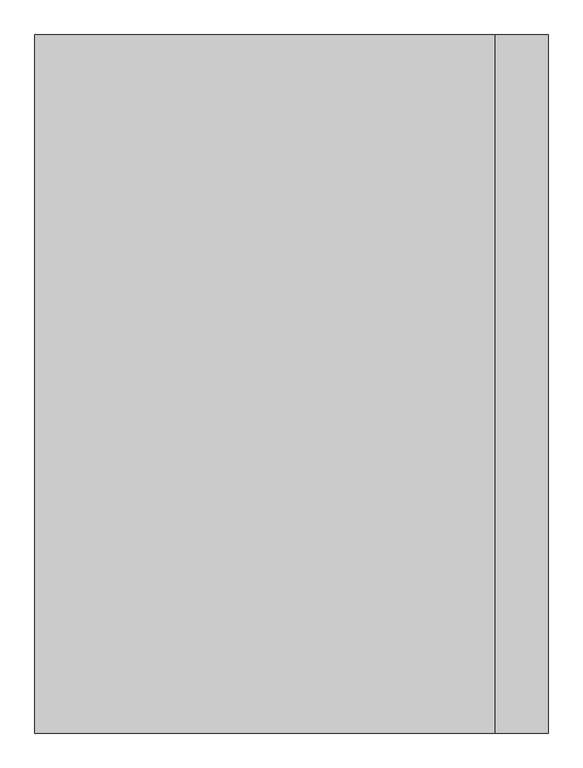
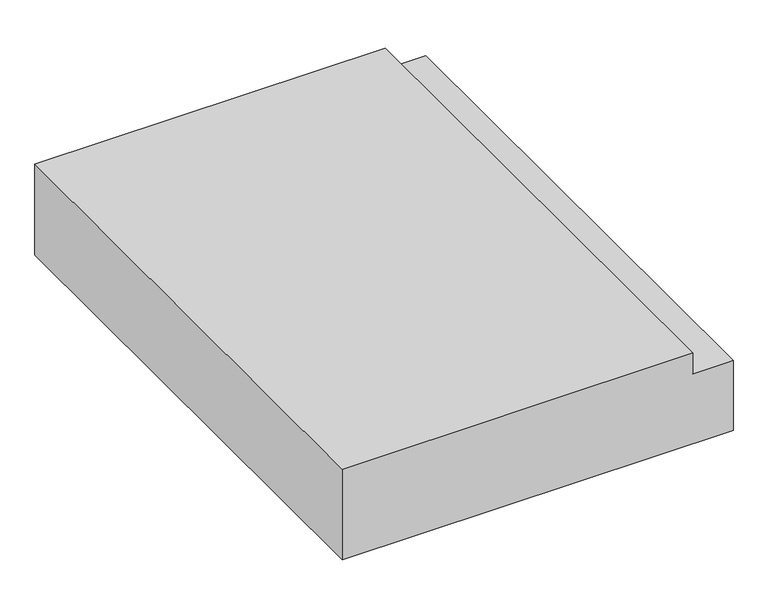
"""IFC4 building model written with IfcOpenShell, lengths in millimetres: proxy geometry, Gravel003 307 : Gravel003 307."""

from ifc_helpers import new_model, si_unit, frame, origin, place, context, project, spatial, polyline, outline, extrude, source, transform, mapped, element, save


def generic_models_56ee6a12(model_context):
    return source(origin(), model_context, "Body", "SweptSolid", [
        extrude(outline(polyline([(32036.6025286, -10098.4737014), (32314.8961275, -10098.4737014), (32314.8961275, -10250.8737014), (32397.0602473, -10250.8737014), (32397.0602473, -11568.4300809), (32036.6025286, -11568.4300809), (32036.6025286, -10098.4737014)])), frame((0.0, 7982.1531721, 0.0), z_axis=(0.0, 1.0, 0.0), x_axis=(0.0, 0.0, 1.0)), (0.0, 0.0, 1.0), 2000.0),
    ])


if __name__ == "__main__":
    model = new_model("IFC4")
    model_context = context("Model", 3, world=origin())
    ifc_project = project(units=[si_unit("LENGTHUNIT", "METRE", prefix="MILLI")], contexts=[model_context])
    site = spatial("IfcSite", under=ifc_project)
    building = spatial("IfcBuilding", under=site)
    placement = place(None, origin())
    generic_models_shape = generic_models_56ee6a12(model_context)
    element("IfcBuildingElementProxy", 1, Name="Gravel003 307 : Gravel003 307", ObjectType="Gravel003 307 : Gravel003 307", at=placement, inside=building, context=model_context, shape_type="MappedRepresentation", body=[
        mapped(generic_models_shape, transform((0.0, 0.0, 0.0), x_axis=(1.0, 0.0, 0.0), y_axis=(0.0, 1.0, 0.0), z_axis=(0.0, 0.0, 1.0))),
    ])
    save(model, "model.ifc")

# Revit data of these elements
# Type "Gravel003 307 : Gravel003 307"
#   NameOverride = "Gravel003"
# Element 1 (IfcBuildingElementProxy, "Gravel003 307 : Gravel003 307")
#   Materials on its faces: "4\" MIN. CRUSHED GRAVEL (NO FINES)"
# Materials
#   "4\" MIN. CRUSHED GRAVEL (NO FINES)": class "Unassigned", colour RGB 145 162 188, transparency 0, Cost = 0
